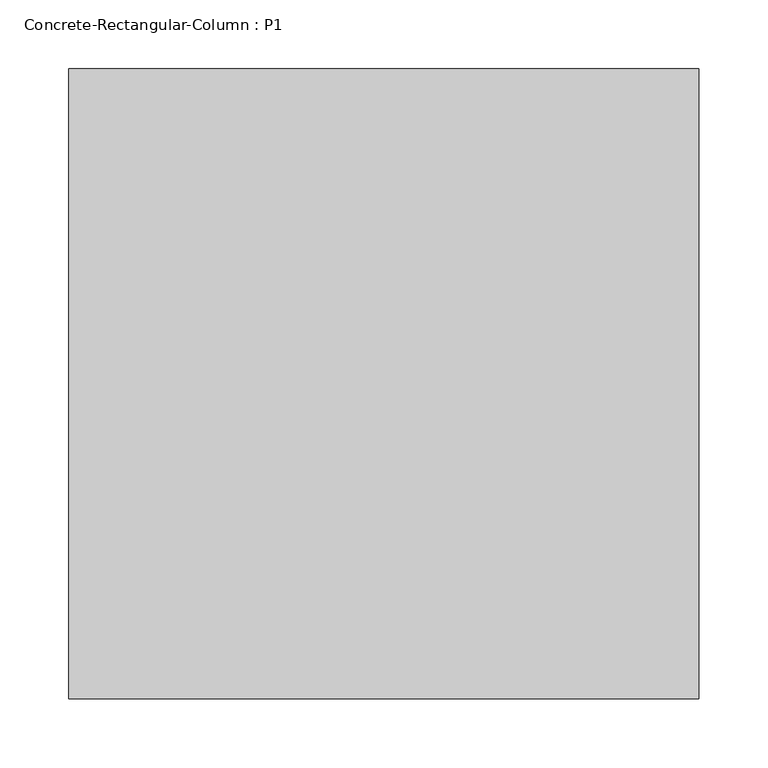
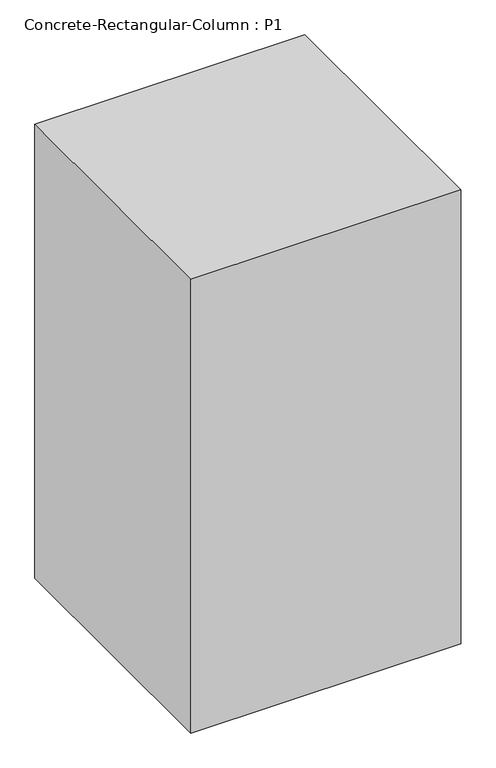
"""IFC4 building model written with IfcOpenShell, lengths in millimetres: column geometry, Concrete-Rectangular-Column : P1."""

from ifc_helpers import new_model, si_unit, frame, origin, place, context, project, spatial, polyline, outline, extrude, source, transform, mapped, element, save


def concrete_rectangular_column_p1_6b068ede(model_context):
    return source(origin(), model_context, "Body", "SweptSolid", [
        extrude(outline(polyline([(228.6, 228.6), (228.6, -228.6), (-228.6, -228.6), (-228.6, 228.6), (228.6, 228.6)])), frame((0.0, 0.0, -812.8), z_axis=(0.0, 0.0, 1.0), x_axis=(1.0, 0.0, 0.0)), (0.0, 0.0, 1.0), 812.8),
    ])


if __name__ == "__main__":
    model = new_model("IFC4")
    model_context = context("Model", 3, world=origin())
    ifc_project = project(units=[si_unit("LENGTHUNIT", "METRE", prefix="MILLI")], contexts=[model_context])
    site = spatial("IfcSite", under=ifc_project)
    building = spatial("IfcBuilding", under=site)
    placement = place(None, origin())
    concrete_rectangular_column_p1_shape = concrete_rectangular_column_p1_6b068ede(model_context)
    element("IfcColumn", 1, ObjectType="Concrete-Rectangular-Column : P1", at=placement, inside=building, context=model_context, shape_type="MappedRepresentation", body=[
        mapped(concrete_rectangular_column_p1_shape, transform((0.0, 0.0, 0.0), x_axis=(1.0, 0.0, 0.0), y_axis=(0.0, 1.0, 0.0), z_axis=(0.0, 0.0, 1.0))),
    ])
    save(model, "model.ifc")

# Revit data of these elements
# Type "Concrete-Rectangular-Column : P1"
#   Assembly Code = "B10"
#   b = 1' - 6"
#   h = 1' - 6"
#   Structural Material [instance default] = Concrete, Cast-in-Place gray
# Element 1 (IfcColumn, "Concrete-Rectangular-Column : P1")
#   Materials on its faces: "Concrete, Cast-in-Place gray"
# Materials
#   "Concrete, Cast-in-Place gray": class "Concrete", colour RGB 192 192 192, transparency 0, Description = "Cast-in-place concrete", Cost = 0
